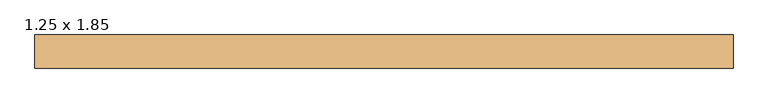
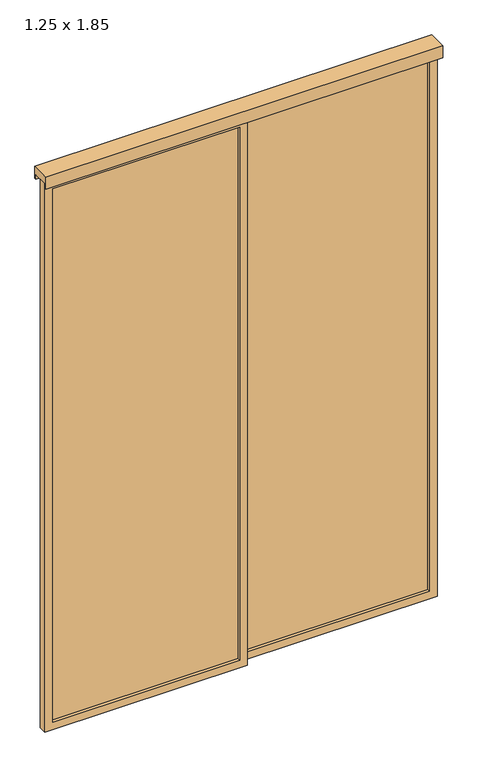
"""IFC4 building model written with IfcOpenShell, lengths in millimetres: door geometry, CC_ND-200_BOX-BANHEIRO : 1.25 x 1.85."""

import ifcopenshell
import ifcopenshell.guid

model = None  # the IFC model being written
_history = None  # IfcOwnerHistory: only IFC2X3 demands one
_inside = {}  # id of a spatial element -> (the spatial element, [elements in it])
_under = {}  # id of a project, library or spatial element -> (it, [spatial elements below it])
_declared = {}  # id of a project -> (the project, [libraries it declares])
_typed = {}  # id of a type object -> (the type object, [elements of that type])
_made_of = {}  # id of a material, layer set ... -> (it, [elements and type objects made of it])


def new_model(schema):
    """Start an empty IFC model of exactly this schema.

    Asked for "IFC4X3", IfcOpenShell would pick the latest addendum, in which some entities
    have other attributes; the version numbers below select the first issue.
    IFC2X3 requires an IfcOwnerHistory on every rooted entity: one is made here for all.
    """
    global model, _history
    if schema == "IFC4X3":
        model = ifcopenshell.file(schema_version=(4, 3, 0, 0))
    else:
        model = ifcopenshell.file(schema=schema)
    _inside.clear()
    _under.clear()
    _declared.clear()
    _typed.clear()
    _made_of.clear()
    _history = None
    if model.schema == "IFC2X3":
        org = make("IfcOrganization", Name="unknown")
        user = make(
            "IfcPersonAndOrganization",
            ThePerson=make("IfcPerson", FamilyName="unknown"),
            TheOrganization=org,
        )
        app = make(
            "IfcApplication",
            ApplicationDeveloper=org,
            Version="unknown",
            ApplicationFullName="unknown",
            ApplicationIdentifier="unknown",
        )
        _history = make(
            "IfcOwnerHistory",
            OwningUser=user,
            OwningApplication=app,
            ChangeAction="ADDED",
            CreationDate=0,
        )
    return model


def make(cls, **values):
    """One entity of the class cls with the attributes given. An attribute that is None is left unset."""
    return model.create_entity(
        cls, **{name: value for name, value in values.items() if value is not None}
    )


def rooted(cls, **values):
    """An entity with a GlobalId (a new one), such as an element, a storey or a relation."""
    return make(cls, GlobalId=ifcopenshell.guid.new(), OwnerHistory=_history, **values)


def si_unit(unit_type, name, prefix=None):
    """IfcSIUnit, for example si_unit("LENGTHUNIT", "METRE", prefix="MILLI")."""
    return make("IfcSIUnit", UnitType=unit_type, Prefix=prefix, Name=name)


def assignment(units):
    """IfcUnitAssignment: the units of a project."""
    return None if units is None else make("IfcUnitAssignment", Units=units)


def point(xyz):
    """IfcCartesianPoint."""
    return None if xyz is None else make("IfcCartesianPoint", Coordinates=xyz)


def direction(xyz):
    """IfcDirection."""
    return None if xyz is None else make("IfcDirection", DirectionRatios=xyz)


def frame(location, z_axis=None, x_axis=None):
    """IfcAxis2Placement3D, a coordinate frame: its origin and axes. An axis left out is left unset."""
    return make(
        "IfcAxis2Placement3D",
        Location=point(location),
        Axis=direction(z_axis),
        RefDirection=direction(x_axis),
    )


def origin():
    """The frame at (0, 0, 0) with its axes left unset."""
    return frame((0.0, 0.0, 0.0))


def place(relative_to, where):
    """IfcLocalPlacement: puts the frame where relative to a parent placement (None: the world)."""
    return make(
        "IfcLocalPlacement", PlacementRelTo=relative_to, RelativePlacement=where
    )


def context(
    kind, dimensions, precision=None, world=None, true_north=None, identifier=None
):
    """IfcGeometricRepresentationContext, for example the 3D "Model" context."""
    return make(
        "IfcGeometricRepresentationContext",
        ContextIdentifier=identifier,
        ContextType=kind,
        CoordinateSpaceDimension=dimensions,
        Precision=precision,
        WorldCoordinateSystem=world,
        TrueNorth=true_north,
    )


def project(units=None, contexts=None):
    """IfcProject with its units and contexts."""
    return rooted(
        "IfcProject",
        Name="project",
        RepresentationContexts=contexts,
        UnitsInContext=assignment(units),
    )


def spatial(cls, under=None, at=None, **own):
    """A site, building, storey or space (cls), placed at a placement, below another one or the project."""
    s = rooted(cls, ObjectPlacement=at, **own)
    if under is not None:
        _under.setdefault(under.id(), (under, []))[1].append(s)
    return s


def polyline(points):
    """IfcPolyline through the points."""
    return make("IfcPolyline", Points=[point(p) for p in points])


def outline(outer, holes=None, kind="AREA"):
    """IfcArbitraryClosedProfileDef: a profile drawn as a closed curve; with holes, ...WithVoids."""
    if holes is None:
        return make("IfcArbitraryClosedProfileDef", ProfileType=kind, OuterCurve=outer)
    return make(
        "IfcArbitraryProfileDefWithVoids",
        ProfileType=kind,
        OuterCurve=outer,
        InnerCurves=holes,
    )


def extrude(swept, where, along, depth):
    """IfcExtrudedAreaSolid: the profile swept, set in the frame where, extruded along a direction by depth."""
    return make(
        "IfcExtrudedAreaSolid",
        SweptArea=swept,
        Position=where,
        ExtrudedDirection=direction(along),
        Depth=depth,
    )


def faces_of(points, faces, orient=None, outer=None):
    """IfcFace entities. A face is a list of loops; a loop is a list of indices into points, from 0.

    orient and outer hold one flag for each loop. By default every Orientation is true, the
    first loop of a face is its IfcFaceOuterBound and the others are IfcFaceBound.
    """
    made = []
    for i, loops in enumerate(faces):
        bounds = []
        for j, loop in enumerate(loops):
            is_outer = j == 0 if outer is None else outer[i][j]
            bounds.append(
                make(
                    "IfcFaceOuterBound" if is_outer else "IfcFaceBound",
                    Bound=make("IfcPolyLoop", Polygon=[points[k] for k in loop]),
                    Orientation=True if orient is None else orient[i][j],
                )
            )
        made.append(make("IfcFace", Bounds=bounds))
    return made


def faceted_brep(points, faces, orient=None, outer=None, voids=None):
    """IfcFacetedBrep: a solid bounded by flat faces; with voids (closed shells), ...WithVoids."""
    shared = [point(p) for p in points]
    hull = make("IfcClosedShell", CfsFaces=faces_of(shared, faces, orient, outer))
    if voids is None:
        return make("IfcFacetedBrep", Outer=hull)
    return make(
        "IfcFacetedBrepWithVoids",
        Outer=hull,
        Voids=[
            make(cls, CfsFaces=faces_of(shared, fs, o, b)) for cls, fs, o, b in voids
        ],
    )


def shape(context_of_items, identifier, shape_type, items):
    """IfcShapeRepresentation: the items that make up one representation, for example the "Body"."""
    return make(
        "IfcShapeRepresentation",
        ContextOfItems=context_of_items,
        RepresentationIdentifier=identifier,
        RepresentationType=shape_type,
        Items=items,
    )


def source(mapping_origin, context_of_items, identifier, shape_type, items):
    """IfcRepresentationMap: a shape defined once, which mapped items show again and again."""
    return make(
        "IfcRepresentationMap",
        MappingOrigin=mapping_origin,
        MappedRepresentation=shape(context_of_items, identifier, shape_type, items),
    )


def transform(
    local_origin,
    x_axis=None,
    y_axis=None,
    z_axis=None,
    scale=None,
    scale2=None,
    scale3=None,
    uniform=True,
):
    """IfcCartesianTransformationOperator3D, or its non-uniform kind. x_axis, y_axis, z_axis: its Axis1, 2, 3."""
    if uniform:
        return make(
            "IfcCartesianTransformationOperator3D",
            Axis1=direction(x_axis),
            Axis2=direction(y_axis),
            LocalOrigin=point(local_origin),
            Scale=scale,
            Axis3=direction(z_axis),
        )
    return make(
        "IfcCartesianTransformationOperator3DnonUniform",
        Axis1=direction(x_axis),
        Axis2=direction(y_axis),
        LocalOrigin=point(local_origin),
        Scale=scale,
        Axis3=direction(z_axis),
        Scale2=scale2,
        Scale3=scale3,
    )


def mapped(mapping_source, mapping_target):
    """IfcMappedItem: shows the shape of a source again, moved by a transform."""
    return make(
        "IfcMappedItem", MappingSource=mapping_source, MappingTarget=mapping_target
    )


def made_of(thing, what):
    """Note that an element or type object is made of a material, layer set ...; save() writes the relation."""
    if what is not None:
        _made_of.setdefault(what.id(), (what, []))[1].append(thing)
    return thing


def element(
    cls,
    number,
    at=None,
    inside=None,
    cuts=None,
    type_object=None,
    material=None,
    context=None,
    identifier="Body",
    shape_type=None,
    held_by="IfcProductDefinitionShape",
    body=None,
    shapes=None,
    **own,
):
    """One element of the class cls, such as IfcWall. Its Tag is "e" and its number.

    at: its placement. inside: the storey or other place that contains it. cuts: it is an
    opening in that element (IfcRelVoidsElement). A single representation is given by context,
    identifier, shape_type and body (its items); several are given by shapes. held_by: the class
    of the entity that holds the representations. save() writes the other relations.
    """
    e = rooted(cls, Tag="e%d" % number, ObjectPlacement=at, **own)
    if body is not None:
        shapes = [shape(context, identifier, shape_type, body)]
    if shapes is not None:
        e.Representation = make(held_by, Representations=shapes)
    if inside is not None:
        _inside.setdefault(inside.id(), (inside, []))[1].append(e)
    if cuts is not None:
        rooted(
            "IfcRelVoidsElement", RelatingBuildingElement=cuts, RelatedOpeningElement=e
        )
    if type_object is not None:
        _typed.setdefault(type_object.id(), (type_object, []))[1].append(e)
    return made_of(e, material)


def aggregate(whole, parts):
    """IfcRelAggregates: a whole, such as a stair, and the parts it consists of."""
    return rooted("IfcRelAggregates", RelatingObject=whole, RelatedObjects=parts)


def save(model, path):
    """Write the relations noted so far, then the file.

    IfcRelAggregates (storeys below a building ...), IfcRelContainedInSpatialStructure (elements
    in a storey), IfcRelDefinesByType, IfcRelAssociatesMaterial and IfcRelDeclares: one each for
    every whole, place, type object, material and project.
    """
    for whole, parts in _under.values():
        aggregate(whole, parts)
    for where, things in _inside.values():
        rooted(
            "IfcRelContainedInSpatialStructure",
            RelatedElements=things,
            RelatingStructure=where,
        )
    for kind, things in _typed.values():
        rooted("IfcRelDefinesByType", RelatedObjects=things, RelatingType=kind)
    for what, things in _made_of.values():
        rooted("IfcRelAssociatesMaterial", RelatedObjects=things, RelatingMaterial=what)
    for by, libraries in _declared.values():
        rooted("IfcRelDeclares", RelatingContext=by, RelatedDefinitions=libraries)
    model.write(path)


def door_1_25_x_1_85_04f1ac89(model_context):
    return source(origin(), model_context, "Body", "SolidModel", [
        extrude(outline(polyline([(627.5, 15.0), (627.5, 10.0), (10.0, 10.0), (10.0, 15.0), (627.5, 15.0)])), frame((0.0, 0.0, 10.0), z_axis=(0.0, 0.0, 1.0), x_axis=(1.0, 0.0, 0.0)), (0.0, 0.0, 1.0), 1805.0),
        faceted_brep([(612.5, 15.0, 1800.0), (612.5, 25.0, 1800.0), (612.5, 25.0, 25.0), (612.5, 15.0, 25.0), (637.5, 25.0, 1825.0), (637.5, 25.0, 0.0), (0.0, 25.0, 0.0), (0.0, 25.0, 1825.0), (25.0, 25.0, 1800.0), (25.0, 25.0, 25.0), (25.0, 15.0, 25.0), (10.0, 15.0, 1815.0), (10.0, 15.0, 10.0), (627.5, 15.0, 10.0), (627.5, 15.0, 1815.0), (25.0, 15.0, 1800.0), (637.5, 0.0, 1825.0), (637.5, 0.0, 0.0), (0.0, 0.0, 1825.0), (0.0, 0.0, 0.0), (612.5, 0.0, 1800.0), (612.5, 0.0, 25.0), (25.0, 0.0, 25.0), (25.0, 0.0, 1800.0), (612.5, 10.0, 1800.0), (612.5, 10.0, 25.0), (25.0, 10.0, 25.0), (25.0, 10.0, 1800.0), (627.5, 10.0, 1815.0), (627.5, 10.0, 10.0), (10.0, 10.0, 10.0), (10.0, 10.0, 1815.0)], [[[0, 1, 2, 3]], [[4, 5, 6, 7], [8, 9, 2, 1]], [[3, 2, 9, 10]], [[11, 12, 13, 14], [0, 3, 10, 15]], [[4, 16, 17, 5]], [[18, 19, 17, 16], [20, 21, 22, 23]], [[5, 17, 19, 6]], [[10, 9, 8, 15]], [[6, 19, 18, 7]], [[20, 24, 25, 21]], [[21, 25, 26, 22]], [[22, 26, 27, 23]], [[28, 14, 13, 29]], [[29, 13, 12, 30]], [[28, 29, 30, 31], [27, 26, 25, 24]], [[30, 12, 11, 31]], [[15, 8, 1, 0]], [[7, 18, 16, 4]], [[31, 11, 14, 28]], [[23, 27, 24, 20]]]),
        extrude(outline(polyline([(1240.0, 40.0), (1240.0, 35.0), (622.5, 35.0), (622.5, 40.0), (1240.0, 40.0)])), frame((0.0, 0.0, 10.0), z_axis=(0.0, 0.0, 1.0), x_axis=(1.0, 0.0, 0.0)), (0.0, 0.0, 1.0), 1805.0),
        faceted_brep([(1225.0, 40.0, 1800.0), (1225.0, 50.0, 1800.0), (1225.0, 50.0, 25.0), (1225.0, 40.0, 25.0), (1250.0, 50.0, 1825.0), (1250.0, 50.0, 0.0), (612.5, 50.0, 0.0), (612.5, 50.0, 1825.0), (637.5, 50.0, 1800.0), (637.5, 50.0, 25.0), (637.5, 40.0, 25.0), (622.5, 40.0, 1815.0), (622.5, 40.0, 10.0), (1240.0, 40.0, 10.0), (1240.0, 40.0, 1815.0), (637.5, 40.0, 1800.0), (1250.0, 25.0, 1825.0), (1250.0, 25.0, 0.0), (612.5, 25.0, 1825.0), (612.5, 25.0, 0.0), (1225.0, 25.0, 1800.0), (1225.0, 25.0, 25.0), (637.5, 25.0, 25.0), (637.5, 25.0, 1800.0), (1225.0, 35.0, 1800.0), (1225.0, 35.0, 25.0), (637.5, 35.0, 25.0), (637.5, 35.0, 1800.0), (1240.0, 35.0, 1815.0), (1240.0, 35.0, 10.0), (622.5, 35.0, 10.0), (622.5, 35.0, 1815.0)], [[[0, 1, 2, 3]], [[4, 5, 6, 7], [8, 9, 2, 1]], [[3, 2, 9, 10]], [[11, 12, 13, 14], [0, 3, 10, 15]], [[4, 16, 17, 5]], [[18, 19, 17, 16], [20, 21, 22, 23]], [[5, 17, 19, 6]], [[10, 9, 8, 15]], [[6, 19, 18, 7]], [[20, 24, 25, 21]], [[21, 25, 26, 22]], [[22, 26, 27, 23]], [[28, 14, 13, 29]], [[29, 13, 12, 30]], [[28, 29, 30, 31], [27, 26, 25, 24]], [[30, 12, 11, 31]], [[15, 8, 1, 0]], [[7, 18, 16, 4]], [[31, 11, 14, 28]], [[23, 27, 24, 20]]]),
        extrude(outline(polyline([(-5.0, 1810.0), (-5.0, 1850.0), (55.0, 1850.0), (55.0, 1810.0), (50.0, 1810.0), (50.0, 1825.0), (0.0, 1825.0), (0.0, 1810.0), (-5.0, 1810.0)])), frame((0.0, 0.0, 0.0), z_axis=(1.0, 0.0, 0.0), x_axis=(0.0, 1.0, 0.0)), (0.0, 0.0, 1.0), 1250.0),
    ])


if __name__ == "__main__":
    model = new_model("IFC4")
    model_context = context("Model", 3, world=origin())
    ifc_project = project(units=[si_unit("LENGTHUNIT", "METRE", prefix="MILLI")], contexts=[model_context])
    site = spatial("IfcSite", under=ifc_project)
    building = spatial("IfcBuilding", under=site)
    placement = place(None, origin())
    door_1_25_x_1_85_shape = door_1_25_x_1_85_04f1ac89(model_context)
    element("IfcDoor", 1, ObjectType="CC_ND-200_BOX-BANHEIRO : 1.25 x 1.85", at=placement, inside=building, context=model_context, shape_type="MappedRepresentation", body=[
        mapped(door_1_25_x_1_85_shape, transform((0.0, 0.0, 0.0), x_axis=(1.0, 0.0, 0.0), y_axis=(0.0, 1.0, 0.0), z_axis=(0.0, 0.0, 1.0))),
    ])
    save(model, "model.ifc")

# Revit data of these elements
# Type "CC_ND-200_BOX-BANHEIRO : 1.25 x 1.85"
#   Type Mark = "150"
#   Width = 1.25 m
#   Material montante = Aluminio
#   Materia vidro = Vidro
# Element 1 (IfcDoor, "CC_ND-200_BOX-BANHEIRO : 1.25 x 1.85")
#   Materials on its faces: "Aluminio", "Vidro"
# Materials
#   "Aluminio": class "Genérico", colour RGB 120 120 120, transparency 0, Cost = 0
#   "Vidro": class "Vidro", colour RGB 230 230 230, transparency 0.75, Description = "JANELA COM 04 FOLHAS DE CORRER E VIDRO TRANSPARENTE 6mm", Cost = 0
